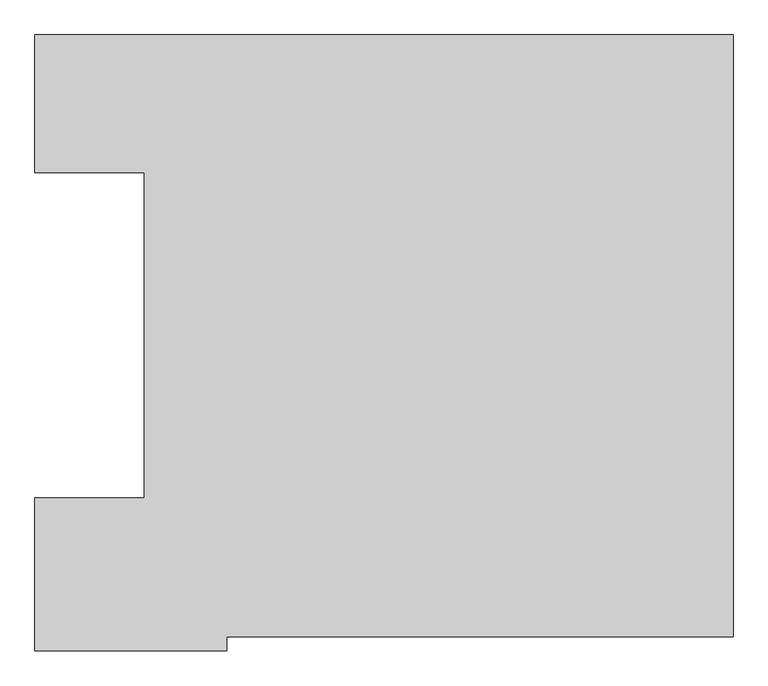
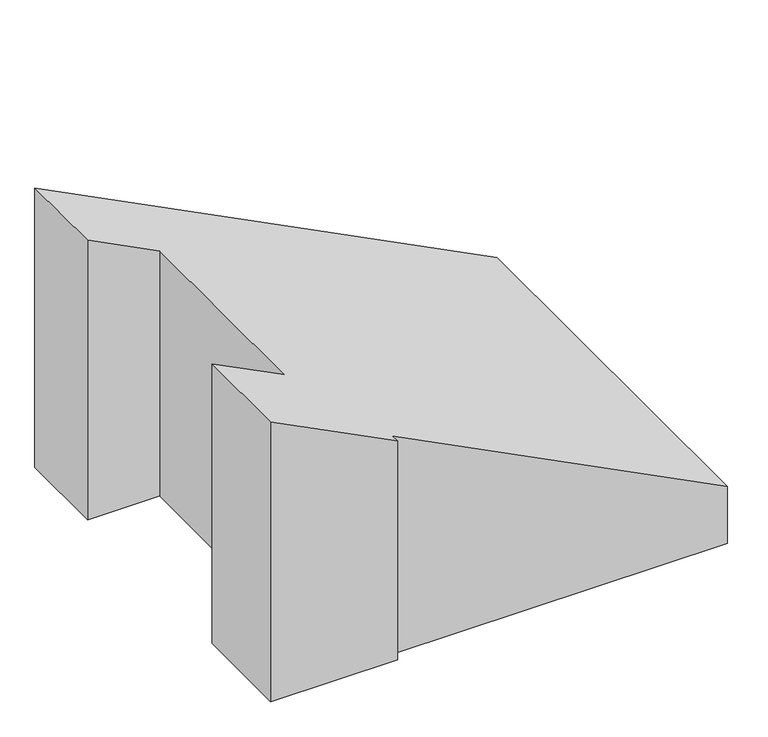
"""IFC4 building model written with IfcOpenShell, lengths in millimetres: proxy geometry, 0_3d_modell."""

from ifc_helpers import new_model, si_unit, origin, place, context, project, spatial, faceted_brep, source, transform, mapped, element, save


def generic_models_7c63ce79(model_context):
    return source(origin(), model_context, "Body", "Brep", [
        faceted_brep([(1025.0, 1435.0, 3668.4620158), (0.0, 1435.0, 4190.7256015), (0.0, 0.0, 4190.7256015), (1800.0, 0.0, 3273.5797924), (1800.0, 130.0, 3273.5797924), (6550.0, 130.0, 853.3339073), (6550.0, 5780.0, 853.3339073), (0.0, 5780.0, 4190.7256015), (0.0, 4487.8, 4190.7256015), (1025.0, 4487.8, 3668.4620158), (6550.0, 130.0, 0.0), (6550.0, 5780.0, 0.0), (1800.0, 130.0, 0.0), (1800.0, 0.0, 0.0), (0.0, 0.0, 0.0), (1025.0, 1435.0, 0.0), (0.0, 1435.0, 0.0), (1025.0, 4487.8, 0.0), (0.0, 4487.8, 0.0), (0.0, 5780.0, 0.0)], [[[0, 1, 2, 3, 4, 5, 6, 7, 8, 9]], [[6, 5, 10, 11]], [[5, 4, 12, 10]], [[4, 3, 13, 12]], [[3, 2, 14, 13]], [[1, 0, 15, 16]], [[0, 9, 17, 15]], [[9, 8, 18, 17]], [[19, 18, 8, 7]], [[7, 6, 11, 19]], [[16, 14, 2, 1]], [[14, 16, 15, 17, 18, 19, 11, 10, 12, 13]]]),
    ])


if __name__ == "__main__":
    model = new_model("IFC4")
    model_context = context("Model", 3, world=origin())
    ifc_project = project(units=[si_unit("LENGTHUNIT", "METRE", prefix="MILLI")], contexts=[model_context])
    site = spatial("IfcSite", under=ifc_project)
    building = spatial("IfcBuilding", under=site)
    placement = place(None, origin())
    generic_models_shape = generic_models_7c63ce79(model_context)
    element("IfcBuildingElementProxy", 1, Name="0_3d_modell", ObjectType="0_3d_modell", at=placement, inside=building, context=model_context, shape_type="MappedRepresentation", body=[
        mapped(generic_models_shape, transform((0.0, 0.0, 0.0), x_axis=(1.0, 0.0, 0.0), y_axis=(0.0, 1.0, 0.0), z_axis=(0.0, 0.0, 1.0))),
    ])
    save(model, "model.ifc")

# Revit data of these elements
# Element 1 (IfcBuildingElementProxy, "0_3d_modell")
#   Materials on its faces: "*1"
# Materials
#   "*1": class "Unassigned", colour RGB 175 175 175, transparency 0
